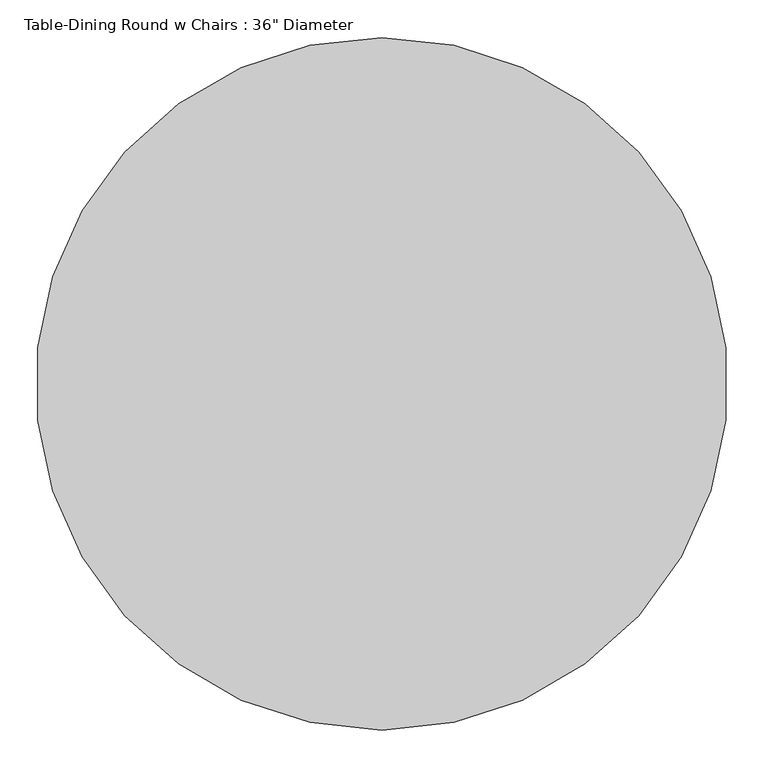
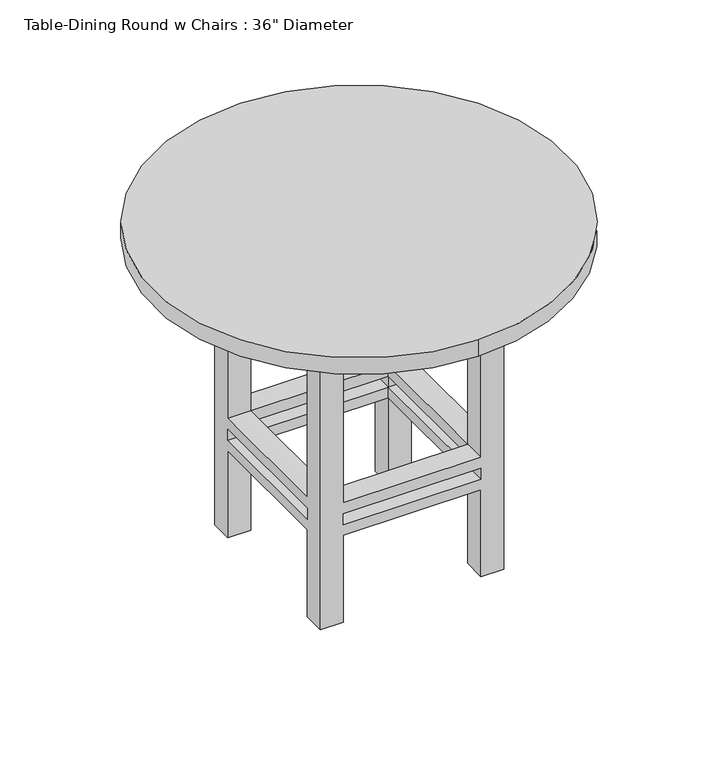
"""IFC4 building model written with IfcOpenShell, lengths in millimetres: furniture geometry."""

import ifcopenshell
import ifcopenshell.guid

model = None  # the IFC model being written
_history = None  # IfcOwnerHistory: only IFC2X3 demands one
_inside = {}  # id of a spatial element -> (the spatial element, [elements in it])
_under = {}  # id of a project, library or spatial element -> (it, [spatial elements below it])
_declared = {}  # id of a project -> (the project, [libraries it declares])
_typed = {}  # id of a type object -> (the type object, [elements of that type])
_made_of = {}  # id of a material, layer set ... -> (it, [elements and type objects made of it])


def new_model(schema):
    """Start an empty IFC model of exactly this schema.

    Asked for "IFC4X3", IfcOpenShell would pick the latest addendum, in which some entities
    have other attributes; the version numbers below select the first issue.
    IFC2X3 requires an IfcOwnerHistory on every rooted entity: one is made here for all.
    """
    global model, _history
    if schema == "IFC4X3":
        model = ifcopenshell.file(schema_version=(4, 3, 0, 0))
    else:
        model = ifcopenshell.file(schema=schema)
    _inside.clear()
    _under.clear()
    _declared.clear()
    _typed.clear()
    _made_of.clear()
    _history = None
    if model.schema == "IFC2X3":
        org = make("IfcOrganization", Name="unknown")
        user = make(
            "IfcPersonAndOrganization",
            ThePerson=make("IfcPerson", FamilyName="unknown"),
            TheOrganization=org,
        )
        app = make(
            "IfcApplication",
            ApplicationDeveloper=org,
            Version="unknown",
            ApplicationFullName="unknown",
            ApplicationIdentifier="unknown",
        )
        _history = make(
            "IfcOwnerHistory",
            OwningUser=user,
            OwningApplication=app,
            ChangeAction="ADDED",
            CreationDate=0,
        )
    return model


def make(cls, **values):
    """One entity of the class cls with the attributes given. An attribute that is None is left unset."""
    return model.create_entity(
        cls, **{name: value for name, value in values.items() if value is not None}
    )


def rooted(cls, **values):
    """An entity with a GlobalId (a new one), such as an element, a storey or a relation."""
    return make(cls, GlobalId=ifcopenshell.guid.new(), OwnerHistory=_history, **values)


def si_unit(unit_type, name, prefix=None):
    """IfcSIUnit, for example si_unit("LENGTHUNIT", "METRE", prefix="MILLI")."""
    return make("IfcSIUnit", UnitType=unit_type, Prefix=prefix, Name=name)


def assignment(units):
    """IfcUnitAssignment: the units of a project."""
    return None if units is None else make("IfcUnitAssignment", Units=units)


def point(xyz):
    """IfcCartesianPoint."""
    return None if xyz is None else make("IfcCartesianPoint", Coordinates=xyz)


def direction(xyz):
    """IfcDirection."""
    return None if xyz is None else make("IfcDirection", DirectionRatios=xyz)


def frame(location, z_axis=None, x_axis=None):
    """IfcAxis2Placement3D, a coordinate frame: its origin and axes. An axis left out is left unset."""
    return make(
        "IfcAxis2Placement3D",
        Location=point(location),
        Axis=direction(z_axis),
        RefDirection=direction(x_axis),
    )


def frame_2d(location, x_axis=None):
    """IfcAxis2Placement2D, a coordinate frame in the plane: its origin and x axis."""
    return make(
        "IfcAxis2Placement2D", Location=point(location), RefDirection=direction(x_axis)
    )


def origin():
    """The frame at (0, 0, 0) with its axes left unset."""
    return frame((0.0, 0.0, 0.0))


def place(relative_to, where):
    """IfcLocalPlacement: puts the frame where relative to a parent placement (None: the world)."""
    return make(
        "IfcLocalPlacement", PlacementRelTo=relative_to, RelativePlacement=where
    )


def context(
    kind, dimensions, precision=None, world=None, true_north=None, identifier=None
):
    """IfcGeometricRepresentationContext, for example the 3D "Model" context."""
    return make(
        "IfcGeometricRepresentationContext",
        ContextIdentifier=identifier,
        ContextType=kind,
        CoordinateSpaceDimension=dimensions,
        Precision=precision,
        WorldCoordinateSystem=world,
        TrueNorth=true_north,
    )


def project(units=None, contexts=None):
    """IfcProject with its units and contexts."""
    return rooted(
        "IfcProject",
        Name="project",
        RepresentationContexts=contexts,
        UnitsInContext=assignment(units),
    )


def spatial(cls, under=None, at=None, **own):
    """A site, building, storey or space (cls), placed at a placement, below another one or the project."""
    s = rooted(cls, ObjectPlacement=at, **own)
    if under is not None:
        _under.setdefault(under.id(), (under, []))[1].append(s)
    return s


def polyline(points):
    """IfcPolyline through the points."""
    return make("IfcPolyline", Points=[point(p) for p in points])


def circle_curve(where, radius):
    """IfcCircle in the frame where."""
    return make("IfcCircle", Position=where, Radius=radius)


def trimmed(basis, trim1, trim2, sense, master):
    """IfcTrimmedCurve: the piece of a basis curve between two trims."""
    return make(
        "IfcTrimmedCurve",
        BasisCurve=basis,
        Trim1=trim1,
        Trim2=trim2,
        SenseAgreement=sense,
        MasterRepresentation=master,
    )


def segment(curve, same_sense, transition):
    """IfcCompositeCurveSegment."""
    return make(
        "IfcCompositeCurveSegment",
        Transition=transition,
        SameSense=same_sense,
        ParentCurve=curve,
    )


def composite_curve(segments, self_intersect=None):
    """IfcCompositeCurve: segments joined end to end."""
    return make("IfcCompositeCurve", Segments=segments, SelfIntersect=self_intersect)


def outline(outer, holes=None, kind="AREA"):
    """IfcArbitraryClosedProfileDef: a profile drawn as a closed curve; with holes, ...WithVoids."""
    if holes is None:
        return make("IfcArbitraryClosedProfileDef", ProfileType=kind, OuterCurve=outer)
    return make(
        "IfcArbitraryProfileDefWithVoids",
        ProfileType=kind,
        OuterCurve=outer,
        InnerCurves=holes,
    )


def extrude(swept, where, along, depth):
    """IfcExtrudedAreaSolid: the profile swept, set in the frame where, extruded along a direction by depth."""
    return make(
        "IfcExtrudedAreaSolid",
        SweptArea=swept,
        Position=where,
        ExtrudedDirection=direction(along),
        Depth=depth,
    )


def faces_of(points, faces, orient=None, outer=None):
    """IfcFace entities. A face is a list of loops; a loop is a list of indices into points, from 0.

    orient and outer hold one flag for each loop. By default every Orientation is true, the
    first loop of a face is its IfcFaceOuterBound and the others are IfcFaceBound.
    """
    made = []
    for i, loops in enumerate(faces):
        bounds = []
        for j, loop in enumerate(loops):
            is_outer = j == 0 if outer is None else outer[i][j]
            bounds.append(
                make(
                    "IfcFaceOuterBound" if is_outer else "IfcFaceBound",
                    Bound=make("IfcPolyLoop", Polygon=[points[k] for k in loop]),
                    Orientation=True if orient is None else orient[i][j],
                )
            )
        made.append(make("IfcFace", Bounds=bounds))
    return made


def faceted_brep(points, faces, orient=None, outer=None, voids=None):
    """IfcFacetedBrep: a solid bounded by flat faces; with voids (closed shells), ...WithVoids."""
    shared = [point(p) for p in points]
    hull = make("IfcClosedShell", CfsFaces=faces_of(shared, faces, orient, outer))
    if voids is None:
        return make("IfcFacetedBrep", Outer=hull)
    return make(
        "IfcFacetedBrepWithVoids",
        Outer=hull,
        Voids=[
            make(cls, CfsFaces=faces_of(shared, fs, o, b)) for cls, fs, o, b in voids
        ],
    )


def shape(context_of_items, identifier, shape_type, items):
    """IfcShapeRepresentation: the items that make up one representation, for example the "Body"."""
    return make(
        "IfcShapeRepresentation",
        ContextOfItems=context_of_items,
        RepresentationIdentifier=identifier,
        RepresentationType=shape_type,
        Items=items,
    )


def source(mapping_origin, context_of_items, identifier, shape_type, items):
    """IfcRepresentationMap: a shape defined once, which mapped items show again and again."""
    return make(
        "IfcRepresentationMap",
        MappingOrigin=mapping_origin,
        MappedRepresentation=shape(context_of_items, identifier, shape_type, items),
    )


def transform(
    local_origin,
    x_axis=None,
    y_axis=None,
    z_axis=None,
    scale=None,
    scale2=None,
    scale3=None,
    uniform=True,
):
    """IfcCartesianTransformationOperator3D, or its non-uniform kind. x_axis, y_axis, z_axis: its Axis1, 2, 3."""
    if uniform:
        return make(
            "IfcCartesianTransformationOperator3D",
            Axis1=direction(x_axis),
            Axis2=direction(y_axis),
            LocalOrigin=point(local_origin),
            Scale=scale,
            Axis3=direction(z_axis),
        )
    return make(
        "IfcCartesianTransformationOperator3DnonUniform",
        Axis1=direction(x_axis),
        Axis2=direction(y_axis),
        LocalOrigin=point(local_origin),
        Scale=scale,
        Axis3=direction(z_axis),
        Scale2=scale2,
        Scale3=scale3,
    )


def mapped(mapping_source, mapping_target):
    """IfcMappedItem: shows the shape of a source again, moved by a transform."""
    return make(
        "IfcMappedItem", MappingSource=mapping_source, MappingTarget=mapping_target
    )


def made_of(thing, what):
    """Note that an element or type object is made of a material, layer set ...; save() writes the relation."""
    if what is not None:
        _made_of.setdefault(what.id(), (what, []))[1].append(thing)
    return thing


def element(
    cls,
    number,
    at=None,
    inside=None,
    cuts=None,
    type_object=None,
    material=None,
    context=None,
    identifier="Body",
    shape_type=None,
    held_by="IfcProductDefinitionShape",
    body=None,
    shapes=None,
    **own,
):
    """One element of the class cls, such as IfcWall. Its Tag is "e" and its number.

    at: its placement. inside: the storey or other place that contains it. cuts: it is an
    opening in that element (IfcRelVoidsElement). A single representation is given by context,
    identifier, shape_type and body (its items); several are given by shapes. held_by: the class
    of the entity that holds the representations. save() writes the other relations.
    """
    e = rooted(cls, Tag="e%d" % number, ObjectPlacement=at, **own)
    if body is not None:
        shapes = [shape(context, identifier, shape_type, body)]
    if shapes is not None:
        e.Representation = make(held_by, Representations=shapes)
    if inside is not None:
        _inside.setdefault(inside.id(), (inside, []))[1].append(e)
    if cuts is not None:
        rooted(
            "IfcRelVoidsElement", RelatingBuildingElement=cuts, RelatedOpeningElement=e
        )
    if type_object is not None:
        _typed.setdefault(type_object.id(), (type_object, []))[1].append(e)
    return made_of(e, material)


def aggregate(whole, parts):
    """IfcRelAggregates: a whole, such as a stair, and the parts it consists of."""
    return rooted("IfcRelAggregates", RelatingObject=whole, RelatedObjects=parts)


def save(model, path):
    """Write the relations noted so far, then the file.

    IfcRelAggregates (storeys below a building ...), IfcRelContainedInSpatialStructure (elements
    in a storey), IfcRelDefinesByType, IfcRelAssociatesMaterial and IfcRelDeclares: one each for
    every whole, place, type object, material and project.
    """
    for whole, parts in _under.values():
        aggregate(whole, parts)
    for where, things in _inside.values():
        rooted(
            "IfcRelContainedInSpatialStructure",
            RelatedElements=things,
            RelatingStructure=where,
        )
    for kind, things in _typed.values():
        rooted("IfcRelDefinesByType", RelatedObjects=things, RelatingType=kind)
    for what, things in _made_of.values():
        rooted("IfcRelAssociatesMaterial", RelatedObjects=things, RelatingMaterial=what)
    for by, libraries in _declared.values():
        rooted("IfcRelDeclares", RelatingContext=by, RelatedDefinitions=libraries)
    model.write(path)


def furniture_905aceb5(model_context):
    return source(origin(), model_context, "Body", "SolidModel", [
        faceted_brep([(256.0819672, -32.4786885, 279.4), (256.0819672, -337.2786885, 279.4), (306.8819672, -337.2786885, 279.4), (306.8819672, -32.4786885, 279.4), (-48.7180328, -337.2786885, 279.4), (-48.7180328, -388.0786885, 279.4), (256.0819672, -388.0786885, 279.4), (-48.7180328, -32.4786885, 279.4), (-99.5180328, -32.4786885, 279.4), (-99.5180328, -337.2786885, 279.4), (256.0819672, 18.3213115, 279.4), (-48.7180328, 18.3213115, 279.4), (256.0819672, -32.4786885, 254.0), (-48.7180328, -32.4786885, 254.0), (-48.7180328, 18.3213115, 254.0), (256.0819672, 18.3213115, 254.0), (-48.7180328, -337.2786885, 254.0), (-99.5180328, -337.2786885, 254.0), (-99.5180328, -32.4786885, 254.0), (256.0819672, -337.2786885, 254.0), (256.0819672, -388.0786885, 254.0), (-48.7180328, -388.0786885, 254.0), (306.8819672, -32.4786885, 254.0), (306.8819672, -337.2786885, 254.0), (-99.5180328, 18.3213115, 647.7), (-48.7180328, 18.3213115, 647.7), (256.0819672, 18.3213115, 647.7), (306.8819672, 18.3213115, 647.7), (306.8819672, 18.3213115, 0.0), (256.0819672, 18.3213115, 0.0), (256.0819672, 18.3213115, 203.2), (-48.7180328, 18.3213115, 203.2), (-48.7180328, 18.3213115, 0.0), (-99.5180328, 18.3213115, 0.0), (-48.7180328, 18.3213115, 228.6), (256.0819672, 18.3213115, 228.6), (-99.5180328, -32.4786885, 647.7), (-99.5180328, -32.4786885, 0.0), (-99.5180328, -32.4786885, 203.2), (-99.5180328, -337.2786885, 203.2), (-99.5180328, -337.2786885, 0.0), (-99.5180328, -388.0786885, 0.0), (-99.5180328, -388.0786885, 647.7), (-99.5180328, -337.2786885, 647.7), (-99.5180328, -337.2786885, 228.6), (-99.5180328, -32.4786885, 228.6), (306.8819672, -388.0786885, 647.7), (256.0819672, -388.0786885, 647.7), (-48.7180328, -388.0786885, 647.7), (-48.7180328, -388.0786885, 0.0), (-48.7180328, -388.0786885, 203.2), (256.0819672, -388.0786885, 203.2), (256.0819672, -388.0786885, 0.0), (306.8819672, -388.0786885, 0.0), (256.0819672, -388.0786885, 228.6), (-48.7180328, -388.0786885, 228.6), (306.8819672, -32.4786885, 647.7), (306.8819672, -337.2786885, 647.7), (306.8819672, -337.2786885, 0.0), (306.8819672, -337.2786885, 203.2), (306.8819672, -32.4786885, 203.2), (306.8819672, -32.4786885, 0.0), (306.8819672, -32.4786885, 228.6), (306.8819672, -337.2786885, 228.6), (-48.7180328, -32.4786885, 647.7), (256.0819672, -337.2786885, 647.7), (256.0819672, -32.4786885, 647.7), (-48.7180328, -337.2786885, 647.7), (256.0819672, -32.4786885, 0.0), (-48.7180328, -337.2786885, 0.0), (-48.7180328, -32.4786885, 0.0), (256.0819672, -337.2786885, 0.0), (-48.7180328, -32.4786885, 228.6), (-48.7180328, -32.4786885, 203.2), (256.0819672, -32.4786885, 228.6), (256.0819672, -32.4786885, 203.2), (256.0819672, -337.2786885, 228.6), (256.0819672, -337.2786885, 203.2), (-48.7180328, -337.2786885, 228.6), (-48.7180328, -337.2786885, 203.2)], [[[0, 1, 2, 3]], [[1, 4, 5, 6]], [[4, 7, 8, 9]], [[7, 0, 10, 11]], [[12, 13, 14, 15]], [[13, 16, 17, 18]], [[16, 19, 20, 21]], [[19, 12, 22, 23]], [[24, 25, 11, 10, 26, 27, 28, 29, 30, 31, 32, 33], [14, 34, 35, 15]], [[36, 24, 33, 37, 38, 39, 40, 41, 42, 43, 9, 8], [17, 44, 45, 18]], [[46, 47, 6, 5, 48, 42, 41, 49, 50, 51, 52, 53], [20, 54, 55, 21]], [[28, 27, 56, 3, 2, 57, 46, 53, 58, 59, 60, 61], [22, 62, 63, 23]], [[1, 0, 12, 19]], [[4, 1, 19, 16]], [[7, 4, 16, 13]], [[0, 7, 13, 12]], [[25, 24, 36, 64]], [[47, 46, 57, 65]], [[26, 66, 56, 27]], [[48, 67, 43, 42]], [[29, 28, 61, 68]], [[49, 41, 40, 69]], [[32, 70, 37, 33]], [[52, 71, 58, 53]], [[13, 18, 45, 72]], [[64, 36, 8, 7]], [[37, 70, 73, 38]], [[14, 13, 72, 34]], [[25, 64, 7, 11]], [[70, 32, 31, 73]], [[12, 15, 35, 74]], [[66, 26, 10, 0]], [[29, 68, 75, 30]], [[22, 12, 74, 62]], [[56, 66, 0, 3]], [[68, 61, 60, 75]], [[19, 23, 63, 76]], [[65, 57, 2, 1]], [[58, 71, 77, 59]], [[20, 19, 76, 54]], [[47, 65, 1, 6]], [[71, 52, 51, 77]], [[16, 21, 55, 78]], [[67, 48, 5, 4]], [[49, 69, 79, 50]], [[17, 16, 78, 44]], [[43, 67, 4, 9]], [[69, 40, 39, 79]], [[74, 76, 63, 62]], [[76, 78, 55, 54]], [[78, 72, 45, 44]], [[72, 74, 35, 34]], [[75, 73, 31, 30]], [[73, 79, 39, 38]], [[79, 77, 51, 50]], [[77, 75, 60, 59]], [[76, 74, 75, 77]], [[78, 76, 77, 79]], [[72, 78, 79, 73]], [[74, 72, 73, 75]]]),
        extrude(outline(polyline([(332.2819672, 43.7213115), (332.2819672, -413.4786885), (-124.9180328, -413.4786885), (-124.9180328, 43.7213115), (332.2819672, 43.7213115)]), holes=[polyline([(306.8819672, 18.3213115), (-99.5180328, 18.3213115), (-99.5180328, -388.0786885), (306.8819672, -388.0786885), (306.8819672, 18.3213115)])]), frame((0.0, 0.0, 647.7), z_axis=(0.0, 0.0, 1.0), x_axis=(1.0, 0.0, 0.0)), (0.0, 0.0, 1.0), 76.2),
        extrude(outline(composite_curve([segment(trimmed(circle_curve(frame_2d((103.6819672, -184.8786885)), 457.2), [point((103.6819672, -642.0786885))], [point((103.6819672, 272.3213115))], False, "CARTESIAN"), True, "CONTINUOUS"), segment(trimmed(circle_curve(frame_2d((103.6819672, -184.8786885)), 457.2), [point((103.6819672, 272.3213115))], [point((103.6819672, -642.0786885))], False, "CARTESIAN"), True, "CONTINUOUS")], self_intersect=False)), frame((0.0, 0.0, 723.9), z_axis=(0.0, 0.0, 1.0), x_axis=(1.0, 0.0, 0.0)), (0.0, 0.0, 1.0), 38.1),
    ])


if __name__ == "__main__":
    model = new_model("IFC4")
    model_context = context("Model", 3, world=origin())
    ifc_project = project(units=[si_unit("LENGTHUNIT", "METRE", prefix="MILLI")], contexts=[model_context])
    site = spatial("IfcSite", under=ifc_project)
    building = spatial("IfcBuilding", under=site)
    placement = place(None, origin())
    furniture_shape = furniture_905aceb5(model_context)
    element("IfcFurniture", 1, ObjectType="Table-Dining Round w Chairs : 36\" Diameter", at=placement, inside=building, context=model_context, shape_type="MappedRepresentation", body=[
        mapped(furniture_shape, transform((0.0, 0.0, 0.0), x_axis=(1.0, 0.0, 0.0), y_axis=(0.0, 1.0, 0.0), z_axis=(0.0, 0.0, 1.0))),
    ])
    save(model, "model.ifc")

# Revit data of these elements
# Type "Table-Dining Round w Chairs : 36\" Diameter"
#   Model = "TBL3456"
#   Manufacturer = "Acme Furniture"
#   Type Mark = "TB-1"
#   Assembly Code = "E2020200"
#   Cost = 375
#   Radius = 1' - 6"
#   Diameter = 3' - 0"
#   Height = 2' - 6"
#   Chairs = 4
#   Base Material = Pine
#   Top Material = Laminate, Linen, Matte
#   Default Elevation = 0
# Element 1 (IfcFurniture, "Table-Dining Round w Chairs : 36\" Diameter")
#   Materials on its faces: "Pine", "Laminate, Linen, Matte"
# Materials
#   "Pine": class "Wood", colour RGB 223 192 134, transparency 0, Description = "Pinus Echinata", Cost = 0
#   "Laminate, Linen, Matte": class "Plastic", colour RGB 249 239 230, transparency 0, Description = "Plastic Laminate - Linen, Matte", Cost = 0
